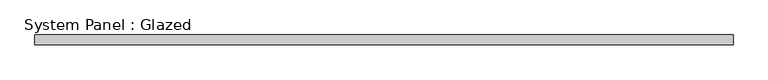
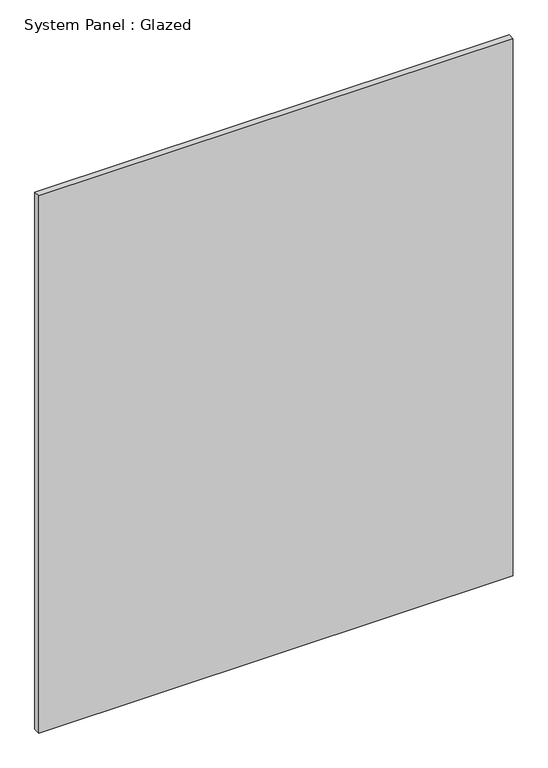
"""IFC4 building model written with IfcOpenShell, lengths in millimetres: plate geometry, System Panel : Glazed."""

import ifcopenshell
import ifcopenshell.guid

model = None  # the IFC model being written
_history = None  # IfcOwnerHistory: only IFC2X3 demands one
_inside = {}  # id of a spatial element -> (the spatial element, [elements in it])
_under = {}  # id of a project, library or spatial element -> (it, [spatial elements below it])
_declared = {}  # id of a project -> (the project, [libraries it declares])
_typed = {}  # id of a type object -> (the type object, [elements of that type])
_made_of = {}  # id of a material, layer set ... -> (it, [elements and type objects made of it])


def new_model(schema):
    """Start an empty IFC model of exactly this schema.

    Asked for "IFC4X3", IfcOpenShell would pick the latest addendum, in which some entities
    have other attributes; the version numbers below select the first issue.
    IFC2X3 requires an IfcOwnerHistory on every rooted entity: one is made here for all.
    """
    global model, _history
    if schema == "IFC4X3":
        model = ifcopenshell.file(schema_version=(4, 3, 0, 0))
    else:
        model = ifcopenshell.file(schema=schema)
    _inside.clear()
    _under.clear()
    _declared.clear()
    _typed.clear()
    _made_of.clear()
    _history = None
    if model.schema == "IFC2X3":
        org = make("IfcOrganization", Name="unknown")
        user = make(
            "IfcPersonAndOrganization",
            ThePerson=make("IfcPerson", FamilyName="unknown"),
            TheOrganization=org,
        )
        app = make(
            "IfcApplication",
            ApplicationDeveloper=org,
            Version="unknown",
            ApplicationFullName="unknown",
            ApplicationIdentifier="unknown",
        )
        _history = make(
            "IfcOwnerHistory",
            OwningUser=user,
            OwningApplication=app,
            ChangeAction="ADDED",
            CreationDate=0,
        )
    return model


def make(cls, **values):
    """One entity of the class cls with the attributes given. An attribute that is None is left unset."""
    return model.create_entity(
        cls, **{name: value for name, value in values.items() if value is not None}
    )


def rooted(cls, **values):
    """An entity with a GlobalId (a new one), such as an element, a storey or a relation."""
    return make(cls, GlobalId=ifcopenshell.guid.new(), OwnerHistory=_history, **values)


def si_unit(unit_type, name, prefix=None):
    """IfcSIUnit, for example si_unit("LENGTHUNIT", "METRE", prefix="MILLI")."""
    return make("IfcSIUnit", UnitType=unit_type, Prefix=prefix, Name=name)


def assignment(units):
    """IfcUnitAssignment: the units of a project."""
    return None if units is None else make("IfcUnitAssignment", Units=units)


def point(xyz):
    """IfcCartesianPoint."""
    return None if xyz is None else make("IfcCartesianPoint", Coordinates=xyz)


def direction(xyz):
    """IfcDirection."""
    return None if xyz is None else make("IfcDirection", DirectionRatios=xyz)


def frame(location, z_axis=None, x_axis=None):
    """IfcAxis2Placement3D, a coordinate frame: its origin and axes. An axis left out is left unset."""
    return make(
        "IfcAxis2Placement3D",
        Location=point(location),
        Axis=direction(z_axis),
        RefDirection=direction(x_axis),
    )


def origin():
    """The frame at (0, 0, 0) with its axes left unset."""
    return frame((0.0, 0.0, 0.0))


def origin_with_axes():
    """The frame at (0, 0, 0) with the z axis (0, 0, 1) and the x axis (1, 0, 0) written out."""
    return frame((0.0, 0.0, 0.0), z_axis=(0.0, 0.0, 1.0), x_axis=(1.0, 0.0, 0.0))


def place(relative_to, where):
    """IfcLocalPlacement: puts the frame where relative to a parent placement (None: the world)."""
    return make(
        "IfcLocalPlacement", PlacementRelTo=relative_to, RelativePlacement=where
    )


def context(
    kind, dimensions, precision=None, world=None, true_north=None, identifier=None
):
    """IfcGeometricRepresentationContext, for example the 3D "Model" context."""
    return make(
        "IfcGeometricRepresentationContext",
        ContextIdentifier=identifier,
        ContextType=kind,
        CoordinateSpaceDimension=dimensions,
        Precision=precision,
        WorldCoordinateSystem=world,
        TrueNorth=true_north,
    )


def project(units=None, contexts=None):
    """IfcProject with its units and contexts."""
    return rooted(
        "IfcProject",
        Name="project",
        RepresentationContexts=contexts,
        UnitsInContext=assignment(units),
    )


def spatial(cls, under=None, at=None, **own):
    """A site, building, storey or space (cls), placed at a placement, below another one or the project."""
    s = rooted(cls, ObjectPlacement=at, **own)
    if under is not None:
        _under.setdefault(under.id(), (under, []))[1].append(s)
    return s


def polyline(points):
    """IfcPolyline through the points."""
    return make("IfcPolyline", Points=[point(p) for p in points])


def outline(outer, holes=None, kind="AREA"):
    """IfcArbitraryClosedProfileDef: a profile drawn as a closed curve; with holes, ...WithVoids."""
    if holes is None:
        return make("IfcArbitraryClosedProfileDef", ProfileType=kind, OuterCurve=outer)
    return make(
        "IfcArbitraryProfileDefWithVoids",
        ProfileType=kind,
        OuterCurve=outer,
        InnerCurves=holes,
    )


def extrude(swept, where, along, depth):
    """IfcExtrudedAreaSolid: the profile swept, set in the frame where, extruded along a direction by depth."""
    return make(
        "IfcExtrudedAreaSolid",
        SweptArea=swept,
        Position=where,
        ExtrudedDirection=direction(along),
        Depth=depth,
    )


def shape(context_of_items, identifier, shape_type, items):
    """IfcShapeRepresentation: the items that make up one representation, for example the "Body"."""
    return make(
        "IfcShapeRepresentation",
        ContextOfItems=context_of_items,
        RepresentationIdentifier=identifier,
        RepresentationType=shape_type,
        Items=items,
    )


def source(mapping_origin, context_of_items, identifier, shape_type, items):
    """IfcRepresentationMap: a shape defined once, which mapped items show again and again."""
    return make(
        "IfcRepresentationMap",
        MappingOrigin=mapping_origin,
        MappedRepresentation=shape(context_of_items, identifier, shape_type, items),
    )


def transform(
    local_origin,
    x_axis=None,
    y_axis=None,
    z_axis=None,
    scale=None,
    scale2=None,
    scale3=None,
    uniform=True,
):
    """IfcCartesianTransformationOperator3D, or its non-uniform kind. x_axis, y_axis, z_axis: its Axis1, 2, 3."""
    if uniform:
        return make(
            "IfcCartesianTransformationOperator3D",
            Axis1=direction(x_axis),
            Axis2=direction(y_axis),
            LocalOrigin=point(local_origin),
            Scale=scale,
            Axis3=direction(z_axis),
        )
    return make(
        "IfcCartesianTransformationOperator3DnonUniform",
        Axis1=direction(x_axis),
        Axis2=direction(y_axis),
        LocalOrigin=point(local_origin),
        Scale=scale,
        Axis3=direction(z_axis),
        Scale2=scale2,
        Scale3=scale3,
    )


def mapped(mapping_source, mapping_target):
    """IfcMappedItem: shows the shape of a source again, moved by a transform."""
    return make(
        "IfcMappedItem", MappingSource=mapping_source, MappingTarget=mapping_target
    )


def made_of(thing, what):
    """Note that an element or type object is made of a material, layer set ...; save() writes the relation."""
    if what is not None:
        _made_of.setdefault(what.id(), (what, []))[1].append(thing)
    return thing


def element(
    cls,
    number,
    at=None,
    inside=None,
    cuts=None,
    type_object=None,
    material=None,
    context=None,
    identifier="Body",
    shape_type=None,
    held_by="IfcProductDefinitionShape",
    body=None,
    shapes=None,
    **own,
):
    """One element of the class cls, such as IfcWall. Its Tag is "e" and its number.

    at: its placement. inside: the storey or other place that contains it. cuts: it is an
    opening in that element (IfcRelVoidsElement). A single representation is given by context,
    identifier, shape_type and body (its items); several are given by shapes. held_by: the class
    of the entity that holds the representations. save() writes the other relations.
    """
    e = rooted(cls, Tag="e%d" % number, ObjectPlacement=at, **own)
    if body is not None:
        shapes = [shape(context, identifier, shape_type, body)]
    if shapes is not None:
        e.Representation = make(held_by, Representations=shapes)
    if inside is not None:
        _inside.setdefault(inside.id(), (inside, []))[1].append(e)
    if cuts is not None:
        rooted(
            "IfcRelVoidsElement", RelatingBuildingElement=cuts, RelatedOpeningElement=e
        )
    if type_object is not None:
        _typed.setdefault(type_object.id(), (type_object, []))[1].append(e)
    return made_of(e, material)


def aggregate(whole, parts):
    """IfcRelAggregates: a whole, such as a stair, and the parts it consists of."""
    return rooted("IfcRelAggregates", RelatingObject=whole, RelatedObjects=parts)


def save(model, path):
    """Write the relations noted so far, then the file.

    IfcRelAggregates (storeys below a building ...), IfcRelContainedInSpatialStructure (elements
    in a storey), IfcRelDefinesByType, IfcRelAssociatesMaterial and IfcRelDeclares: one each for
    every whole, place, type object, material and project.
    """
    for whole, parts in _under.values():
        aggregate(whole, parts)
    for where, things in _inside.values():
        rooted(
            "IfcRelContainedInSpatialStructure",
            RelatedElements=things,
            RelatingStructure=where,
        )
    for kind, things in _typed.values():
        rooted("IfcRelDefinesByType", RelatedObjects=things, RelatingType=kind)
    for what, things in _made_of.values():
        rooted("IfcRelAssociatesMaterial", RelatedObjects=things, RelatingMaterial=what)
    for by, libraries in _declared.values():
        rooted("IfcRelDeclares", RelatingContext=by, RelatedDefinitions=libraries)
    model.write(path)


def system_panel_glazed_fd736ec2(model_context):
    return source(origin(), model_context, "Body", "SweptSolid", [
        extrude(outline(polyline([(887.9485033, -49.5), (-887.9485033, -49.5), (-887.9485033, -24.5), (887.9485033, -24.5), (887.9485033, -49.5)])), origin_with_axes(), (0.0, 0.0, 1.0), 2125.0),
    ])


if __name__ == "__main__":
    model = new_model("IFC4")
    model_context = context("Model", 3, world=origin())
    ifc_project = project(units=[si_unit("LENGTHUNIT", "METRE", prefix="MILLI")], contexts=[model_context])
    site = spatial("IfcSite", under=ifc_project)
    building = spatial("IfcBuilding", under=site)
    placement = place(None, origin())
    system_panel_glazed_shape = system_panel_glazed_fd736ec2(model_context)
    element("IfcPlate", 1, ObjectType="System Panel : Glazed", at=placement, inside=building, context=model_context, shape_type="MappedRepresentation", body=[
        mapped(system_panel_glazed_shape, transform((0.0, 0.0, 0.0), x_axis=(1.0, 0.0, 0.0), y_axis=(0.0, 1.0, 0.0), z_axis=(0.0, 0.0, 1.0))),
    ])
    save(model, "model.ifc")

# Revit data of these elements
# Type "System Panel : Glazed"
#   Keynote = "H11"
#   Construction Type Id = "GSP4R"
#   Analytic Construction = "1/8 in Pilkington single glazing"
#   Visual Light Transmittance = 0.9
#   Solar Heat Gain Coefficient = 0.86
#   Heat Transfer Coefficient (U) = 6.7069 W/(m²·K)
# Element 1 (IfcPlate, "System Panel : Glazed")
#   Materials on its faces: "Glass"
# Materials
#   "Glass": class "Glass", colour RGB 0 128 192, transparency 0.9, Description = "Soda Lime Glass", Cost = 0
